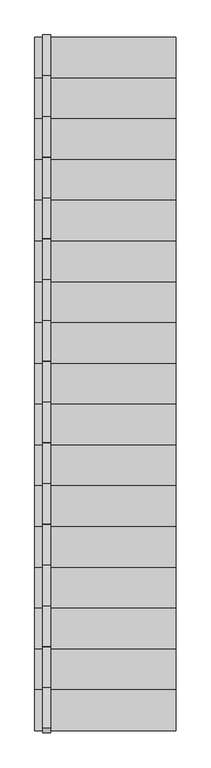
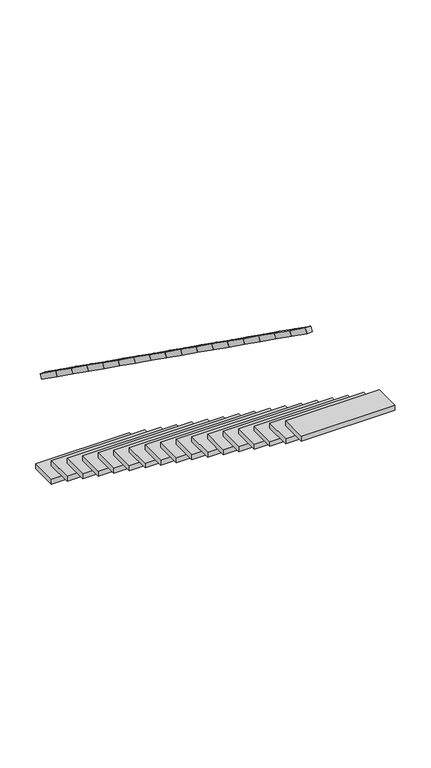
"""IFC4 building model written with IfcOpenShell, lengths in millimetres: stair geometry,   92587 :   92587."""

from ifc_helpers import new_model, si_unit, frame, origin, place, context, project, spatial, polyline, outline, extrude, source, transform, mapped, element, save


def stair_667f7fc2(model_context):
    return source(origin(), model_context, "Body", "SweptSolid", [
        extrude(outline(polyline([(0.0, -319.1002977), (0.0, 0.0), (50.0, 0.0), (50.0, -319.1002977), (0.0, -319.1002977)])), frame((162072.7593015, 34520.3024209, 4178.947508), z_axis=(0.0, 0.5797550216229128, 0.8147908411997622), x_axis=(-1.0, 0.0, 0.0)), (0.0, 0.0, 1.0), 50.0),
        extrude(outline(polyline([(0.0, -319.1002977), (0.0, 0.0), (50.0, 0.0), (50.0, -319.1002977), (0.0, -319.1002977)])), frame((162072.7593015, 34780.3024209, 3993.947508), z_axis=(0.0, 0.5797550216229022, 0.8147908411997696), x_axis=(-1.0, 0.0, 0.0)), (0.0, 0.0, 1.0), 50.0),
        extrude(outline(polyline([(0.0, -319.1002977), (0.0, 0.0), (50.0, 0.0), (50.0, -319.1002977), (0.0, -319.1002977)])), frame((162072.7593015, 35040.3024209, 3808.947508), z_axis=(0.0, 0.5797550216229116, 0.814790841199763), x_axis=(-1.0, 0.0, 0.0)), (0.0, 0.0, 1.0), 50.0),
        extrude(outline(polyline([(0.0, -319.1002977), (0.0, 0.0), (50.0, 0.0), (50.0, -319.1002977), (0.0, -319.1002977)])), frame((162072.7593015, 35300.3024209, 3623.947508), z_axis=(0.0, 0.5797550216229086, 0.8147908411997651), x_axis=(-1.0, 0.0, 0.0)), (0.0, 0.0, 1.0), 50.0),
        extrude(outline(polyline([(0.0, -319.1002977), (0.0, 0.0), (50.0, 0.0), (50.0, -319.1002977), (0.0, -319.1002977)])), frame((162072.7593015, 35560.3024209, 3438.947508), z_axis=(0.0, 0.5797550216229094, 0.8147908411997645), x_axis=(-1.0, 0.0, 0.0)), (0.0, 0.0, 1.0), 50.0),
        extrude(outline(polyline([(0.0, -319.1002977), (0.0, 0.0), (50.0, 0.0), (50.0, -319.1002977), (0.0, -319.1002977)])), frame((162072.7593015, 35820.3024209, 3253.947508), z_axis=(0.0, 0.5797550216228999, 0.8147908411997712), x_axis=(-1.0, 0.0, 0.0)), (0.0, 0.0, 1.0), 50.0),
        extrude(outline(polyline([(0.0, -319.1002977), (0.0, 0.0), (50.0, 0.0), (50.0, -319.1002977), (0.0, -319.1002977)])), frame((162072.7593015, 36080.3024209, 3068.947508), z_axis=(0.0, 0.579755021622915, 0.8147908411997605), x_axis=(-1.0, 0.0, 0.0)), (0.0, 0.0, 1.0), 50.0),
        extrude(outline(polyline([(0.0, -319.1002977), (0.0, 0.0), (50.0, 0.0), (50.0, -319.1002977), (0.0, -319.1002977)])), frame((162072.7593015, 36340.3024209, 2883.947508), z_axis=(0.0, 0.5797550216229139, 0.8147908411997614), x_axis=(-1.0, 0.0, 0.0)), (0.0, 0.0, 1.0), 50.0),
        extrude(outline(polyline([(0.0, -319.1002977), (0.0, 0.0), (50.0, 0.0), (50.0, -319.1002977), (0.0, -319.1002977)])), frame((162072.7593015, 36600.3024209, 2698.947508), z_axis=(0.0, 0.5797550216229128, 0.8147908411997622), x_axis=(-1.0, 0.0, 0.0)), (0.0, 0.0, 1.0), 50.0),
        extrude(outline(polyline([(0.0, -319.1002977), (0.0, 0.0), (50.0, 0.0), (50.0, -319.1002977), (0.0, -319.1002977)])), frame((162072.7593015, 36860.3024209, 2513.947508), z_axis=(0.0, 0.5797550216228966, 0.8147908411997736), x_axis=(-1.0, 0.0, 0.0)), (0.0, 0.0, 1.0), 50.0),
        extrude(outline(polyline([(0.0, -319.1002977), (0.0, 0.0), (50.0, 0.0), (50.0, -319.1002977), (0.0, -319.1002977)])), frame((162072.7593015, 37120.3024209, 2328.947508), z_axis=(0.0, 0.5797550216229123, 0.8147908411997625), x_axis=(-1.0, 0.0, 0.0)), (0.0, 0.0, 1.0), 50.0),
        extrude(outline(polyline([(0.0, -319.1002977), (0.0, 0.0), (50.0, 0.0), (50.0, -319.1002977), (0.0, -319.1002977)])), frame((162072.7593015, 37380.3024209, 2143.947508), z_axis=(0.0, 0.5797550216229139, 0.8147908411997614), x_axis=(-1.0, 0.0, 0.0)), (0.0, 0.0, 1.0), 50.0),
        extrude(outline(polyline([(0.0, -319.1002977), (0.0, 0.0), (50.0, 0.0), (50.0, -319.1002977), (0.0, -319.1002977)])), frame((162072.7593015, 37640.3024209, 1958.947508), z_axis=(0.0, 0.5797550216228999, 0.8147908411997712), x_axis=(-1.0, 0.0, 0.0)), (0.0, 0.0, 1.0), 50.0),
        extrude(outline(polyline([(0.0, -319.1002977), (0.0, 0.0), (50.0, 0.0), (50.0, -319.1002977), (0.0, -319.1002977)])), frame((162072.7593015, 37900.3024209, 1773.947508), z_axis=(0.0, 0.579755021622915, 0.8147908411997605), x_axis=(-1.0, 0.0, 0.0)), (0.0, 0.0, 1.0), 50.0),
        extrude(outline(polyline([(0.0, -319.1002977), (0.0, 0.0), (50.0, 0.0), (50.0, -319.1002977), (0.0, -319.1002977)])), frame((162072.7593015, 38160.3024209, 1588.947508), z_axis=(0.0, 0.579755021622908, 0.8147908411997654), x_axis=(-1.0, 0.0, 0.0)), (0.0, 0.0, 1.0), 50.0),
        extrude(outline(polyline([(0.0, -319.1002977), (0.0, 0.0), (50.0, 0.0), (50.0, -319.1002977), (0.0, -319.1002977)])), frame((162072.7593015, 38420.3024209, 1403.947508), z_axis=(0.0, 0.5797550216229066, 0.8147908411997665), x_axis=(-1.0, 0.0, 0.0)), (0.0, 0.0, 1.0), 50.0),
        extrude(outline(polyline([(0.0, -319.1002977), (0.0, 0.0), (50.0, 0.0), (50.0, -319.1002977), (0.0, -319.1002977)])), frame((162072.7593015, 38680.3024209, 1218.947508), z_axis=(0.0, 0.5797550216228985, 0.8147908411997723), x_axis=(-1.0, 0.0, 0.0)), (0.0, 0.0, 1.0), 50.0),
        extrude(outline(polyline([(161972.7593015, 38694.7962965), (161972.7593015, 38954.7962965), (162872.7593015, 38954.7962965), (162872.7593015, 38694.7962965), (161972.7593015, 38694.7962965)])), frame((0.0, 0.0, 135.0), z_axis=(0.0, 0.0, 1.0), x_axis=(1.0, 0.0, 0.0)), (0.0, 0.0, 1.0), 50.0),
        extrude(outline(polyline([(161972.7593015, 38434.7962965), (161972.7593015, 38694.7962965), (162872.7593015, 38694.7962965), (162872.7593015, 38434.7962965), (161972.7593015, 38434.7962965)])), frame((0.0, 0.0, 320.0), z_axis=(0.0, 0.0, 1.0), x_axis=(1.0, 0.0, 0.0)), (0.0, 0.0, 1.0), 50.0),
        extrude(outline(polyline([(161972.7593015, 38174.7962965), (161972.7593015, 38434.7962965), (162872.7593015, 38434.7962965), (162872.7593015, 38174.7962965), (161972.7593015, 38174.7962965)])), frame((0.0, 0.0, 505.0), z_axis=(0.0, 0.0, 1.0), x_axis=(1.0, 0.0, 0.0)), (0.0, 0.0, 1.0), 50.0),
        extrude(outline(polyline([(161972.7593015, 37914.7962965), (161972.7593015, 38174.7962965), (162872.7593015, 38174.7962965), (162872.7593015, 37914.7962965), (161972.7593015, 37914.7962965)])), frame((0.0, 0.0, 690.0), z_axis=(0.0, 0.0, 1.0), x_axis=(1.0, 0.0, 0.0)), (0.0, 0.0, 1.0), 50.0),
        extrude(outline(polyline([(161972.7593015, 37654.7962965), (161972.7593015, 37914.7962965), (162872.7593015, 37914.7962965), (162872.7593015, 37654.7962965), (161972.7593015, 37654.7962965)])), frame((0.0, 0.0, 875.0), z_axis=(0.0, 0.0, 1.0), x_axis=(1.0, 0.0, 0.0)), (0.0, 0.0, 1.0), 50.0),
        extrude(outline(polyline([(161972.7593015, 37394.7962965), (161972.7593015, 37654.7962965), (162872.7593015, 37654.7962965), (162872.7593015, 37394.7962965), (161972.7593015, 37394.7962965)])), frame((0.0, 0.0, 1060.0), z_axis=(0.0, 0.0, 1.0), x_axis=(1.0, 0.0, 0.0)), (0.0, 0.0, 1.0), 50.0),
        extrude(outline(polyline([(161972.7593015, 37134.7962965), (161972.7593015, 37394.7962965), (162872.7593015, 37394.7962965), (162872.7593015, 37134.7962965), (161972.7593015, 37134.7962965)])), frame((0.0, 0.0, 1245.0), z_axis=(0.0, 0.0, 1.0), x_axis=(1.0, 0.0, 0.0)), (0.0, 0.0, 1.0), 50.0),
        extrude(outline(polyline([(161972.7593015, 36874.7962965), (161972.7593015, 37134.7962965), (162872.7593015, 37134.7962965), (162872.7593015, 36874.7962965), (161972.7593015, 36874.7962965)])), frame((0.0, 0.0, 1430.0), z_axis=(0.0, 0.0, 1.0), x_axis=(1.0, 0.0, 0.0)), (0.0, 0.0, 1.0), 50.0),
        extrude(outline(polyline([(161972.7593015, 36614.7962965), (161972.7593015, 36874.7962965), (162872.7593015, 36874.7962965), (162872.7593015, 36614.7962965), (161972.7593015, 36614.7962965)])), frame((0.0, 0.0, 1615.0), z_axis=(0.0, 0.0, 1.0), x_axis=(1.0, 0.0, 0.0)), (0.0, 0.0, 1.0), 50.0),
        extrude(outline(polyline([(161972.7593015, 36354.7962965), (161972.7593015, 36614.7962965), (162872.7593015, 36614.7962965), (162872.7593015, 36354.7962965), (161972.7593015, 36354.7962965)])), frame((0.0, 0.0, 1800.0), z_axis=(0.0, 0.0, 1.0), x_axis=(1.0, 0.0, 0.0)), (0.0, 0.0, 1.0), 50.0),
        extrude(outline(polyline([(161972.7593015, 36094.7962965), (161972.7593015, 36354.7962965), (162872.7593015, 36354.7962965), (162872.7593015, 36094.7962965), (161972.7593015, 36094.7962965)])), frame((0.0, 0.0, 1985.0), z_axis=(0.0, 0.0, 1.0), x_axis=(1.0, 0.0, 0.0)), (0.0, 0.0, 1.0), 50.0),
        extrude(outline(polyline([(161972.7593015, 35834.7962965), (161972.7593015, 36094.7962965), (162872.7593015, 36094.7962965), (162872.7593015, 35834.7962965), (161972.7593015, 35834.7962965)])), frame((0.0, 0.0, 2170.0), z_axis=(0.0, 0.0, 1.0), x_axis=(1.0, 0.0, 0.0)), (0.0, 0.0, 1.0), 50.0),
        extrude(outline(polyline([(161972.7593015, 35574.7962965), (161972.7593015, 35834.7962965), (162872.7593015, 35834.7962965), (162872.7593015, 35574.7962965), (161972.7593015, 35574.7962965)])), frame((0.0, 0.0, 2355.0), z_axis=(0.0, 0.0, 1.0), x_axis=(1.0, 0.0, 0.0)), (0.0, 0.0, 1.0), 50.0),
        extrude(outline(polyline([(161972.7593015, 35314.7962965), (161972.7593015, 35574.7962965), (162872.7593015, 35574.7962965), (162872.7593015, 35314.7962965), (161972.7593015, 35314.7962965)])), frame((0.0, 0.0, 2540.0), z_axis=(0.0, 0.0, 1.0), x_axis=(1.0, 0.0, 0.0)), (0.0, 0.0, 1.0), 50.0),
        extrude(outline(polyline([(161972.7593015, 35054.7962965), (161972.7593015, 35314.7962965), (162872.7593015, 35314.7962965), (162872.7593015, 35054.7962965), (161972.7593015, 35054.7962965)])), frame((0.0, 0.0, 2725.0), z_axis=(0.0, 0.0, 1.0), x_axis=(1.0, 0.0, 0.0)), (0.0, 0.0, 1.0), 50.0),
        extrude(outline(polyline([(161972.7593015, 34794.7962965), (161972.7593015, 35054.7962965), (162872.7593015, 35054.7962965), (162872.7593015, 34794.7962965), (161972.7593015, 34794.7962965)])), frame((0.0, 0.0, 2910.0), z_axis=(0.0, 0.0, 1.0), x_axis=(1.0, 0.0, 0.0)), (0.0, 0.0, 1.0), 50.0),
        extrude(outline(polyline([(161972.7593015, 34534.7962965), (161972.7593015, 34794.7962965), (162872.7593015, 34794.7962965), (162872.7593015, 34534.7962965), (161972.7593015, 34534.7962965)])), frame((0.0, 0.0, 3095.0), z_axis=(0.0, 0.0, 1.0), x_axis=(1.0, 0.0, 0.0)), (0.0, 0.0, 1.0), 50.0),
    ])


if __name__ == "__main__":
    model = new_model("IFC4")
    model_context = context("Model", 3, world=origin())
    ifc_project = project(units=[si_unit("LENGTHUNIT", "METRE", prefix="MILLI")], contexts=[model_context])
    site = spatial("IfcSite", under=ifc_project)
    building = spatial("IfcBuilding", under=site)
    placement = place(None, origin())
    stair_shape = stair_667f7fc2(model_context)
    element("IfcStair", 1, ObjectType="  92587 :   92587", at=placement, inside=building, context=model_context, shape_type="MappedRepresentation", body=[
        mapped(stair_shape, transform((0.0, 0.0, 0.0), x_axis=(1.0, 0.0, 0.0), y_axis=(0.0, 1.0, 0.0), z_axis=(0.0, 0.0, 1.0))),
    ])
    save(model, "model.ifc")

# Revit data of these elements
# Type "  92587 :   92587"
#   Abrechnungsart = "St"
#   Allright_Bauteil_ID = "0121Tre0785067483"
#   Material = "Stahlbeton"
#   Objektname = "Treppe"
#   NameOverride = " "
#   ThermalTransmittance = 0.0000 BTU/(h·ft²·°F)
#   NosingLength = 0.000 m
#   NumberOfRiser = 18
#   NumberOfTreads = 17
#   RiserHeight = 1.850 m
#   TreadLength = 2.600 m
#   IsExternal = no
#   FireExit = no
#   HandicapAccessible = no
#   HasNonSkidSurface = no
# Element 1 (IfcStair, "  92587 :   92587")
#   Materials on its faces: "*1", "weiss"
# Materials
#   "*1": class "Unassigned", colour RGB 175 175 175, transparency 0
#   "weiss": class "Unassigned", colour RGB 255 255 255, transparency 0
